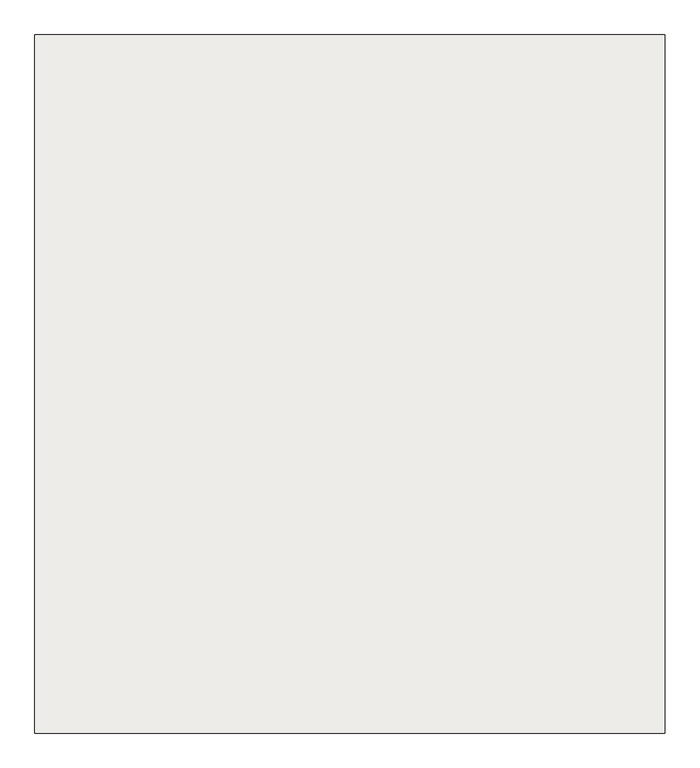
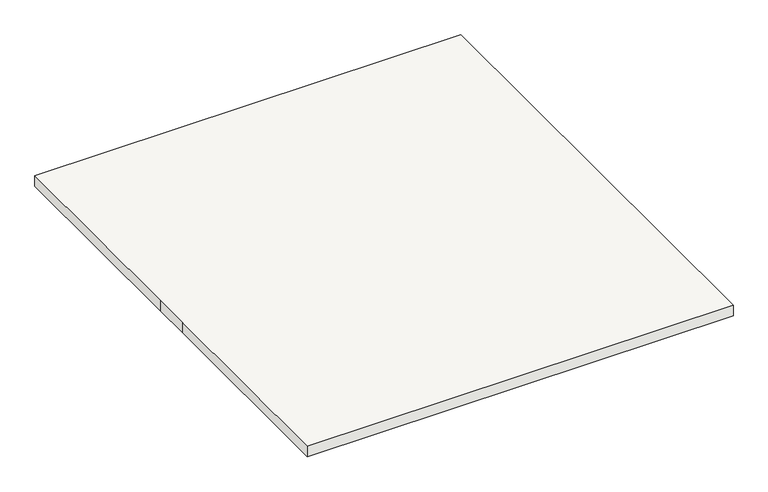
"""IFC4 building model written with IfcOpenShell, lengths in millimetres: slab geometry."""

import ifcopenshell
import ifcopenshell.guid

model = None  # the IFC model being written
_history = None  # IfcOwnerHistory: only IFC2X3 demands one
_inside = {}  # id of a spatial element -> (the spatial element, [elements in it])
_under = {}  # id of a project, library or spatial element -> (it, [spatial elements below it])
_declared = {}  # id of a project -> (the project, [libraries it declares])
_typed = {}  # id of a type object -> (the type object, [elements of that type])
_made_of = {}  # id of a material, layer set ... -> (it, [elements and type objects made of it])


def new_model(schema):
    """Start an empty IFC model of exactly this schema.

    Asked for "IFC4X3", IfcOpenShell would pick the latest addendum, in which some entities
    have other attributes; the version numbers below select the first issue.
    IFC2X3 requires an IfcOwnerHistory on every rooted entity: one is made here for all.
    """
    global model, _history
    if schema == "IFC4X3":
        model = ifcopenshell.file(schema_version=(4, 3, 0, 0))
    else:
        model = ifcopenshell.file(schema=schema)
    _inside.clear()
    _under.clear()
    _declared.clear()
    _typed.clear()
    _made_of.clear()
    _history = None
    if model.schema == "IFC2X3":
        org = make("IfcOrganization", Name="unknown")
        user = make(
            "IfcPersonAndOrganization",
            ThePerson=make("IfcPerson", FamilyName="unknown"),
            TheOrganization=org,
        )
        app = make(
            "IfcApplication",
            ApplicationDeveloper=org,
            Version="unknown",
            ApplicationFullName="unknown",
            ApplicationIdentifier="unknown",
        )
        _history = make(
            "IfcOwnerHistory",
            OwningUser=user,
            OwningApplication=app,
            ChangeAction="ADDED",
            CreationDate=0,
        )
    return model


def make(cls, **values):
    """One entity of the class cls with the attributes given. An attribute that is None is left unset."""
    return model.create_entity(
        cls, **{name: value for name, value in values.items() if value is not None}
    )


def rooted(cls, **values):
    """An entity with a GlobalId (a new one), such as an element, a storey or a relation."""
    return make(cls, GlobalId=ifcopenshell.guid.new(), OwnerHistory=_history, **values)


def si_unit(unit_type, name, prefix=None):
    """IfcSIUnit, for example si_unit("LENGTHUNIT", "METRE", prefix="MILLI")."""
    return make("IfcSIUnit", UnitType=unit_type, Prefix=prefix, Name=name)


def assignment(units):
    """IfcUnitAssignment: the units of a project."""
    return None if units is None else make("IfcUnitAssignment", Units=units)


def point(xyz):
    """IfcCartesianPoint."""
    return None if xyz is None else make("IfcCartesianPoint", Coordinates=xyz)


def direction(xyz):
    """IfcDirection."""
    return None if xyz is None else make("IfcDirection", DirectionRatios=xyz)


def frame(location, z_axis=None, x_axis=None):
    """IfcAxis2Placement3D, a coordinate frame: its origin and axes. An axis left out is left unset."""
    return make(
        "IfcAxis2Placement3D",
        Location=point(location),
        Axis=direction(z_axis),
        RefDirection=direction(x_axis),
    )


def origin():
    """The frame at (0, 0, 0) with its axes left unset."""
    return frame((0.0, 0.0, 0.0))


def place(relative_to, where):
    """IfcLocalPlacement: puts the frame where relative to a parent placement (None: the world)."""
    return make(
        "IfcLocalPlacement", PlacementRelTo=relative_to, RelativePlacement=where
    )


def context(
    kind, dimensions, precision=None, world=None, true_north=None, identifier=None
):
    """IfcGeometricRepresentationContext, for example the 3D "Model" context."""
    return make(
        "IfcGeometricRepresentationContext",
        ContextIdentifier=identifier,
        ContextType=kind,
        CoordinateSpaceDimension=dimensions,
        Precision=precision,
        WorldCoordinateSystem=world,
        TrueNorth=true_north,
    )


def project(units=None, contexts=None):
    """IfcProject with its units and contexts."""
    return rooted(
        "IfcProject",
        Name="project",
        RepresentationContexts=contexts,
        UnitsInContext=assignment(units),
    )


def spatial(cls, under=None, at=None, **own):
    """A site, building, storey or space (cls), placed at a placement, below another one or the project."""
    s = rooted(cls, ObjectPlacement=at, **own)
    if under is not None:
        _under.setdefault(under.id(), (under, []))[1].append(s)
    return s


def polyline(points):
    """IfcPolyline through the points."""
    return make("IfcPolyline", Points=[point(p) for p in points])


def outline(outer, holes=None, kind="AREA"):
    """IfcArbitraryClosedProfileDef: a profile drawn as a closed curve; with holes, ...WithVoids."""
    if holes is None:
        return make("IfcArbitraryClosedProfileDef", ProfileType=kind, OuterCurve=outer)
    return make(
        "IfcArbitraryProfileDefWithVoids",
        ProfileType=kind,
        OuterCurve=outer,
        InnerCurves=holes,
    )


def extrude(swept, where, along, depth):
    """IfcExtrudedAreaSolid: the profile swept, set in the frame where, extruded along a direction by depth."""
    return make(
        "IfcExtrudedAreaSolid",
        SweptArea=swept,
        Position=where,
        ExtrudedDirection=direction(along),
        Depth=depth,
    )


def shape(context_of_items, identifier, shape_type, items):
    """IfcShapeRepresentation: the items that make up one representation, for example the "Body"."""
    return make(
        "IfcShapeRepresentation",
        ContextOfItems=context_of_items,
        RepresentationIdentifier=identifier,
        RepresentationType=shape_type,
        Items=items,
    )


def source(mapping_origin, context_of_items, identifier, shape_type, items):
    """IfcRepresentationMap: a shape defined once, which mapped items show again and again."""
    return make(
        "IfcRepresentationMap",
        MappingOrigin=mapping_origin,
        MappedRepresentation=shape(context_of_items, identifier, shape_type, items),
    )


def transform(
    local_origin,
    x_axis=None,
    y_axis=None,
    z_axis=None,
    scale=None,
    scale2=None,
    scale3=None,
    uniform=True,
):
    """IfcCartesianTransformationOperator3D, or its non-uniform kind. x_axis, y_axis, z_axis: its Axis1, 2, 3."""
    if uniform:
        return make(
            "IfcCartesianTransformationOperator3D",
            Axis1=direction(x_axis),
            Axis2=direction(y_axis),
            LocalOrigin=point(local_origin),
            Scale=scale,
            Axis3=direction(z_axis),
        )
    return make(
        "IfcCartesianTransformationOperator3DnonUniform",
        Axis1=direction(x_axis),
        Axis2=direction(y_axis),
        LocalOrigin=point(local_origin),
        Scale=scale,
        Axis3=direction(z_axis),
        Scale2=scale2,
        Scale3=scale3,
    )


def mapped(mapping_source, mapping_target):
    """IfcMappedItem: shows the shape of a source again, moved by a transform."""
    return make(
        "IfcMappedItem", MappingSource=mapping_source, MappingTarget=mapping_target
    )


def made_of(thing, what):
    """Note that an element or type object is made of a material, layer set ...; save() writes the relation."""
    if what is not None:
        _made_of.setdefault(what.id(), (what, []))[1].append(thing)
    return thing


def element(
    cls,
    number,
    at=None,
    inside=None,
    cuts=None,
    type_object=None,
    material=None,
    context=None,
    identifier="Body",
    shape_type=None,
    held_by="IfcProductDefinitionShape",
    body=None,
    shapes=None,
    **own,
):
    """One element of the class cls, such as IfcWall. Its Tag is "e" and its number.

    at: its placement. inside: the storey or other place that contains it. cuts: it is an
    opening in that element (IfcRelVoidsElement). A single representation is given by context,
    identifier, shape_type and body (its items); several are given by shapes. held_by: the class
    of the entity that holds the representations. save() writes the other relations.
    """
    e = rooted(cls, Tag="e%d" % number, ObjectPlacement=at, **own)
    if body is not None:
        shapes = [shape(context, identifier, shape_type, body)]
    if shapes is not None:
        e.Representation = make(held_by, Representations=shapes)
    if inside is not None:
        _inside.setdefault(inside.id(), (inside, []))[1].append(e)
    if cuts is not None:
        rooted(
            "IfcRelVoidsElement", RelatingBuildingElement=cuts, RelatedOpeningElement=e
        )
    if type_object is not None:
        _typed.setdefault(type_object.id(), (type_object, []))[1].append(e)
    return made_of(e, material)


def aggregate(whole, parts):
    """IfcRelAggregates: a whole, such as a stair, and the parts it consists of."""
    return rooted("IfcRelAggregates", RelatingObject=whole, RelatedObjects=parts)


def save(model, path):
    """Write the relations noted so far, then the file.

    IfcRelAggregates (storeys below a building ...), IfcRelContainedInSpatialStructure (elements
    in a storey), IfcRelDefinesByType, IfcRelAssociatesMaterial and IfcRelDeclares: one each for
    every whole, place, type object, material and project.
    """
    for whole, parts in _under.values():
        aggregate(whole, parts)
    for where, things in _inside.values():
        rooted(
            "IfcRelContainedInSpatialStructure",
            RelatedElements=things,
            RelatingStructure=where,
        )
    for kind, things in _typed.values():
        rooted("IfcRelDefinesByType", RelatedObjects=things, RelatingType=kind)
    for what, things in _made_of.values():
        rooted("IfcRelAssociatesMaterial", RelatedObjects=things, RelatingMaterial=what)
    for by, libraries in _declared.values():
        rooted("IfcRelDeclares", RelatingContext=by, RelatedDefinitions=libraries)
    model.write(path)


def slab_7d48b352(model_context):
    return source(origin(), model_context, "Body", "SweptSolid", [
        extrude(outline(polyline([(5276.5556606, 3685.7983707), (7240.2909543, 3685.7983707), (7240.2909543, 1510.81281), (5276.5556606, 1510.81281), (5276.5556606, 2510.81281), (5276.5556606, 2685.7983707), (5276.5556606, 3685.7983707)])), frame((0.0, 0.0, 1600.0), z_axis=(0.0, 0.0, 1.0), x_axis=(1.0, 0.0, 0.0)), (0.0, 0.0, 1.0), 50.0),
    ])


if __name__ == "__main__":
    model = new_model("IFC4")
    model_context = context("Model", 3, world=origin())
    ifc_project = project(units=[si_unit("LENGTHUNIT", "METRE", prefix="MILLI")], contexts=[model_context])
    site = spatial("IfcSite", under=ifc_project)
    building = spatial("IfcBuilding", under=site)
    placement = place(None, origin())
    slab_shape = slab_7d48b352(model_context)
    element("IfcSlab", 1, at=placement, inside=building, context=model_context, shape_type="MappedRepresentation", body=[
        mapped(slab_shape, transform((0.0, 0.0, 0.0), x_axis=(1.0, 0.0, 0.0), y_axis=(0.0, 1.0, 0.0), z_axis=(0.0, 0.0, 1.0))),
    ])
    save(model, "model.ifc")
